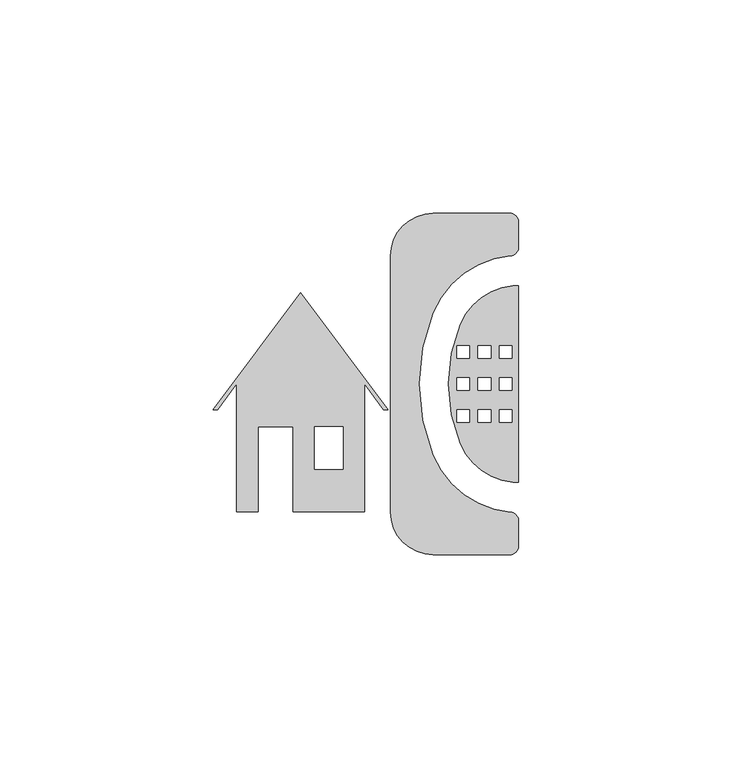
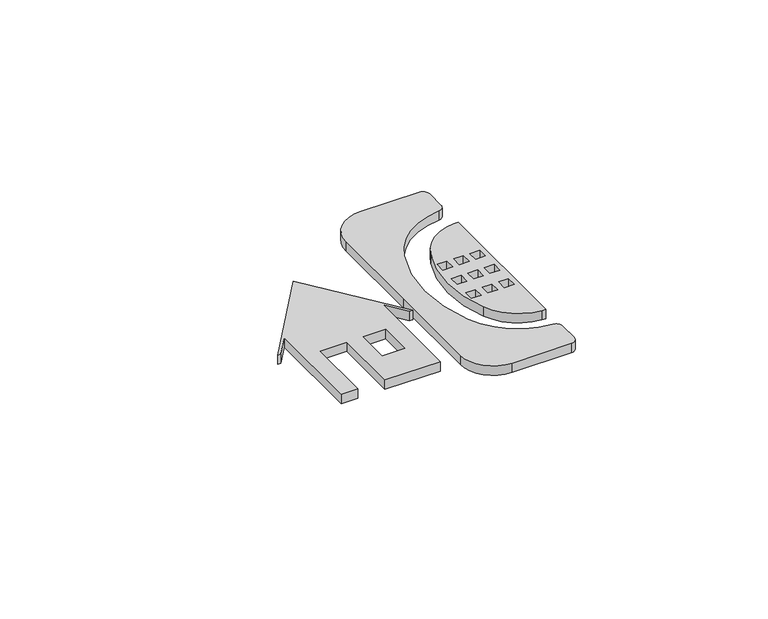
"""IFC4 building model written with IfcOpenShell, lengths in millimetres: proxy geometry, TSP Telkom-connection point external : TSP Telkom-connection point external."""

from ifc_helpers import new_model, si_unit, point, frame_2d, origin, origin_with_axes, place, context, project, spatial, polyline, circle_curve, trimmed, segment, composite_curve, outline, extrude, source, transform, mapped, element, save


def electrical_fixtures_a3c7e1a9(model_context):
    return source(origin(), model_context, "Body", "SweptSolid", [
        extrude(outline(composite_curve([segment(polyline([(0.0, 38.0), (0.0, 32.0)]), True, "CONTINUOUS"), segment(trimmed(circle_curve(frame_2d((-2.0, 32.0)), 2.0), [point((0.0, 32.0))], [point((-1.8374907, 30.0066133))], False, "CARTESIAN"), True, "CONTINUOUS"), segment(trimmed(circle_curve(frame_2d((0.0, 8.4180035)), 21.6666667), [point((-1.8374907, 30.0066133))], [point((-20.0, 16.7513368))], True, "CARTESIAN"), True, "CONTINUOUS"), segment(trimmed(circle_curve(frame_2d((20.2032083, 0.0)), 43.5534757), [point((-20.0, 16.7513368))], [point((-20.0, -16.7513368))], True, "CARTESIAN"), True, "CONTINUOUS"), segment(trimmed(circle_curve(frame_2d((0.0, -8.4180035)), 21.6666667), [point((-20.0, -16.7513368))], [point((-1.8374907, -30.0066133))], True, "CARTESIAN"), True, "CONTINUOUS"), segment(trimmed(circle_curve(frame_2d((-2.0, -32.0)), 2.0), [point((-1.8374907, -30.0066133))], [point((0.0, -32.0))], False, "CARTESIAN"), True, "CONTINUOUS"), segment(polyline([(0.0, -32.0), (0.0, -38.0)]), True, "CONTINUOUS"), segment(trimmed(circle_curve(frame_2d((-2.0, -38.0)), 2.0), [point((0.0, -38.0))], [point((-2.0, -40.0))], False, "CARTESIAN"), True, "CONTINUOUS"), segment(polyline([(-2.0, -40.0), (-20.0, -40.0)]), True, "CONTINUOUS"), segment(trimmed(circle_curve(frame_2d((-20.0, -30.0)), 10.0), [point((-20.0, -40.0))], [point((-30.0, -30.0))], False, "CARTESIAN"), True, "CONTINUOUS"), segment(polyline([(-30.0, -30.0), (-30.0, 0.0), (-30.0, 30.0)]), True, "CONTINUOUS"), segment(trimmed(circle_curve(frame_2d((-20.0, 30.0)), 10.0), [point((-30.0, 30.0))], [point((-20.0, 40.0))], False, "CARTESIAN"), True, "CONTINUOUS"), segment(polyline([(-20.0, 40.0), (-2.0, 40.0)]), True, "CONTINUOUS"), segment(trimmed(circle_curve(frame_2d((-2.0, 38.0)), 2.0), [point((-2.0, 40.0))], [point((0.0, 38.0))], False, "CARTESIAN"), True, "CONTINUOUS")], self_intersect=False)), origin_with_axes(), (0.0, 0.0, 1.0), 3.0),
        extrude(outline(composite_curve([segment(trimmed(circle_curve(frame_2d((20.2032083, 0.0)), 36.5534757), [point((-13.5384615, -14.0590291))], [point((-13.5384615, 14.0590291))], False, "CARTESIAN"), True, "CONTINUOUS"), segment(trimmed(circle_curve(frame_2d((0.0, 8.4180035)), 14.6666667), [point((-13.5384615, 14.0590291))], [point((-1.2438398, 23.0318316))], False, "CARTESIAN"), True, "CONTINUOUS"), segment(polyline([(-1.2438398, 23.0318316), (0.0, 23.0318316), (0.0, -23.0318316), (-1.2438398, -23.0318316)]), True, "CONTINUOUS"), segment(trimmed(circle_curve(frame_2d((0.0, -8.4180035)), 14.6666667), [point((-1.2438398, -23.0318316))], [point((-13.5384615, -14.0590291))], False, "CARTESIAN"), True, "CONTINUOUS")], self_intersect=False), holes=[polyline([(-6.4751337, 9.0), (-9.4524255, 9.0), (-9.4524255, 6.0), (-6.4751337, 6.0), (-6.4751337, 9.0)]), polyline([(-11.4751337, 9.0), (-14.4524255, 9.0), (-14.4524255, 6.0), (-11.4751337, 6.0), (-11.4751337, 9.0)]), polyline([(-4.4751337, 9.0), (-4.4751337, 6.0), (-1.4978419, 6.0), (-1.4978419, 9.0), (-4.4751337, 9.0)]), polyline([(-6.4751337, -9.0), (-6.4751337, -6.0), (-9.4524255, -6.0), (-9.4524255, -9.0), (-6.4751337, -9.0)]), polyline([(-11.4751337, -9.0), (-11.4751337, -6.0), (-14.4524255, -6.0), (-14.4524255, -9.0), (-11.4751337, -9.0)]), polyline([(-4.4751337, -9.0), (-1.4978419, -9.0), (-1.4978419, -6.0), (-4.4751337, -6.0), (-4.4751337, -9.0)]), polyline([(-6.4751337, -1.5), (-6.4751337, 1.5), (-9.4524255, 1.5), (-9.4524255, -1.5), (-6.4751337, -1.5)]), polyline([(-11.4751337, -1.5), (-11.4751337, 1.5), (-14.4524255, 1.5), (-14.4524255, -1.5), (-11.4751337, -1.5)]), polyline([(-4.4751337, -1.5), (-1.4978419, -1.5), (-1.4978419, 1.5), (-4.4751337, 1.5), (-4.4751337, -1.5)])]), origin_with_axes(), (0.0, 0.0, 1.0), 3.0),
        extrude(outline(polyline([(-52.8099378, -30.0), (-52.8099378, -10.0), (-61.0678133, -10.0), (-61.0678133, -30.0), (-66.0678133, -30.0), (-66.0678133, 0.0), (-70.5678133, -6.0), (-71.5678133, -6.0), (-51.0678133, 21.3333333), (-30.5678133, -6.0), (-31.5678133, -6.0), (-36.0678133, 0.0), (-36.0678133, -30.0), (-52.8099378, -30.0)]), holes=[polyline([(-41.0678133, -10.0), (-47.8099378, -10.0), (-47.8099378, -20.0), (-41.0678133, -20.0), (-41.0678133, -10.0)])]), origin_with_axes(), (0.0, 0.0, 1.0), 3.0),
    ])


if __name__ == "__main__":
    model = new_model("IFC4")
    model_context = context("Model", 3, world=origin())
    ifc_project = project(units=[si_unit("LENGTHUNIT", "METRE", prefix="MILLI")], contexts=[model_context])
    site = spatial("IfcSite", under=ifc_project)
    building = spatial("IfcBuilding", under=site)
    placement = place(None, origin())
    electrical_fixtures_shape = electrical_fixtures_a3c7e1a9(model_context)
    element("IfcBuildingElementProxy", 1, Name="TSP Telkom-connection point external : TSP Telkom-connection point external", ObjectType="TSP Telkom-connection point external : TSP Telkom-connection point external", at=placement, inside=building, context=model_context, shape_type="MappedRepresentation", body=[
        mapped(electrical_fixtures_shape, transform((0.0, 0.0, 0.0), x_axis=(1.0, 0.0, 0.0), y_axis=(0.0, 1.0, 0.0), z_axis=(0.0, 0.0, 1.0))),
    ])
    save(model, "model.ifc")

# Revit data of these elements
# Type "TSP Telkom-connection point external : TSP Telkom-connection point external"
#   Model = "TSP_ELECTELPEC"
#   Default Elevation = 0
# Element 1 (IfcBuildingElementProxy, "TSP Telkom-connection point external : TSP Telkom-connection point external")
#   Materials on its faces: "Aluminum, Anodized Red"
# Materials
#   "Aluminum, Anodized Red": class "Metal", colour RGB 120 120 120, transparency 0, Description = "Anodized aluminum, red", Cost = 0
